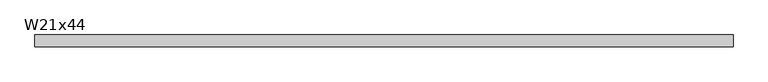
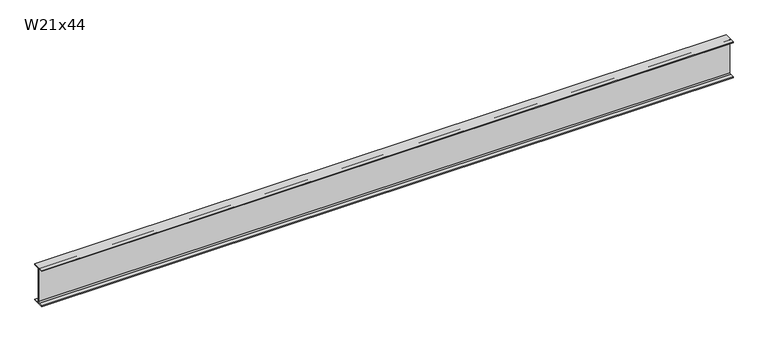
"""IFC4 building model written with IfcOpenShell, lengths in millimetres: beam geometry, RME W-Wide Flange : W21x44."""

from ifc_helpers import new_model, si_unit, point, frame, frame_2d, origin, place, context, project, spatial, polyline, circle_curve, trimmed, segment, composite_curve, outline, extrude, source, transform, mapped, element, save


def w21x44_75b17fcb(model_context):
    return source(origin(), model_context, "Body", "SweptSolid", [
        extrude(outline(composite_curve([segment(polyline([(82.55, -251.46), (82.55, -262.89), (-82.55, -262.89), (-82.55, -251.46), (-21.59, -251.46)]), True, "CONTINUOUS"), segment(trimmed(circle_curve(frame_2d((-21.59, -234.315)), 17.145), [point((-21.59, -251.46))], [point((-4.445, -234.315))], True, "CARTESIAN"), True, "CONTINUOUS"), segment(polyline([(-4.445, -234.315), (-4.445, 234.315)]), True, "CONTINUOUS"), segment(trimmed(circle_curve(frame_2d((-21.59, 234.315)), 17.145), [point((-4.445, 234.315))], [point((-21.59, 251.46))], True, "CARTESIAN"), True, "CONTINUOUS"), segment(polyline([(-21.59, 251.46), (-82.55, 251.46), (-82.55, 262.89), (82.55, 262.89), (82.55, 251.46), (21.59, 251.46)]), True, "CONTINUOUS"), segment(trimmed(circle_curve(frame_2d((21.59, 234.315)), 17.145), [point((21.59, 251.46))], [point((4.445, 234.315))], True, "CARTESIAN"), True, "CONTINUOUS"), segment(polyline([(4.445, 234.315), (4.445, -234.315)]), True, "CONTINUOUS"), segment(trimmed(circle_curve(frame_2d((21.59, -234.315)), 17.145), [point((4.445, -234.315))], [point((21.59, -251.46))], True, "CARTESIAN"), True, "CONTINUOUS"), segment(polyline([(21.59, -251.46), (82.55, -251.46)]), True, "CONTINUOUS")], self_intersect=False)), frame((-4781.55, 0.0, 0.0), z_axis=(1.0, 0.0, 0.0), x_axis=(0.0, 1.0, 0.0)), (0.0, 0.0, 1.0), 9562.592),
    ])


if __name__ == "__main__":
    model = new_model("IFC4")
    model_context = context("Model", 3, world=origin())
    ifc_project = project(units=[si_unit("LENGTHUNIT", "METRE", prefix="MILLI")], contexts=[model_context])
    site = spatial("IfcSite", under=ifc_project)
    building = spatial("IfcBuilding", under=site)
    placement = place(None, origin())
    w21x44_shape = w21x44_75b17fcb(model_context)
    element("IfcBeam", 1, ObjectType="RME W-Wide Flange : W21x44", at=placement, inside=building, context=model_context, shape_type="MappedRepresentation", body=[
        mapped(w21x44_shape, transform((0.0, 0.0, 0.0), x_axis=(1.0, 0.0, 0.0), y_axis=(0.0, 1.0, 0.0), z_axis=(0.0, 0.0, 1.0))),
    ])
    save(model, "model.ifc")

# Revit data of these elements
# Type "RME W-Wide Flange : W21x44"
#   WELD P [instance default] = ""
#   WELD LE [instance default] = ""
#   WELD D [instance default] = ""
#   TOP SECTION SIZE [instance default] = ""
#   TOP SECTION LENGTH [instance default] = ""
#   REMARKS [instance default] = ""
#   REINF TYPE [instance default] = ""
#   Nominal Size = "W24"
#   End Bearing Capacity [instance default] = ""
#   BOT SECTION SIZE [instance default] = ""
#   BOT SECTION LENGTH [instance default] = ""
#   Assembly Code = "B10"
#   W = 44
#   Start Extension Calculation [instance default] = 10' - 0"
#   Start Extension [instance default] = -0' - 0 1/2"
#   End Extension Calculation [instance default] = 10' - 0"
#   End Extension [instance default] = -0' - 0 1/2"
#   Length [instance default] = 5' - 0"
#   bf = 0' - 6 1/2"
#   d = 1' - 8.7"
#   k = 0' - 1 1/8"
#   k2 = 0' - 0.675"
#   tf = 0' - 0.45"
#   tw = 0' - 0.35"
#   A = 0.0902778 SF
#   Structural Material [instance default] = Metal - Steel - ASTM A992
# Element 1 (IfcBeam, "RME W-Wide Flange : W21x44")
#   Length = 32' - 0"
#   Materials on its faces: "Metal - Steel - ASTM A992"
# Materials
#   "Metal - Steel - ASTM A992": class "Metal", colour RGB 255 128 0, transparency 0
